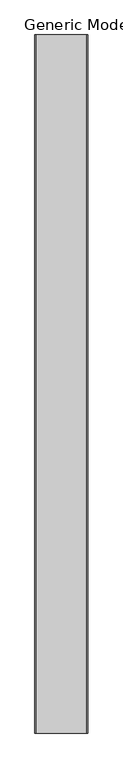
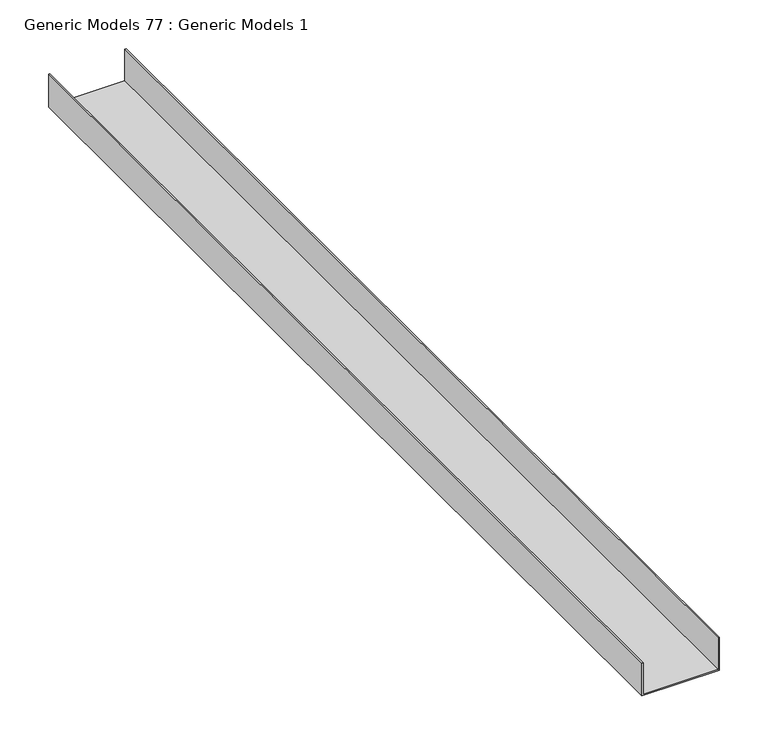
"""IFC4 building model written with IfcOpenShell, lengths in millimetres: proxy geometry, Generic Models 77 : Generic Models 1."""

from ifc_helpers import new_model, si_unit, frame, origin, place, context, project, spatial, polyline, outline, extrude, source, transform, mapped, element, save


def generic_models_77_generic_models_1_8efd1fd8(model_context):
    return source(origin(), model_context, "Body", "SweptSolid", [
        extrude(outline(polyline([(-225.976067, 46935.8735531), (-184.701067, 46935.8735531), (-184.701067, 46934.2860531), (-224.388567, 46934.2860531), (-224.388567, 46845.3860531), (-184.701067, 46845.3860531), (-184.701067, 46843.7985531), (-225.976067, 46843.7985531), (-225.976067, 46935.8735531)])), frame((0.0, 0.0, 0.0), z_axis=(0.0, 1.0, 0.0), x_axis=(0.0, 0.0, 1.0)), (0.0, 0.0, 1.0), 1219.2),
    ])


if __name__ == "__main__":
    model = new_model("IFC4")
    model_context = context("Model", 3, world=origin())
    ifc_project = project(units=[si_unit("LENGTHUNIT", "METRE", prefix="MILLI")], contexts=[model_context])
    site = spatial("IfcSite", under=ifc_project)
    building = spatial("IfcBuilding", under=site)
    placement = place(None, origin())
    generic_models_77_generic_models_1_shape = generic_models_77_generic_models_1_8efd1fd8(model_context)
    element("IfcBuildingElementProxy", 1, Name="Generic Models 77 : Generic Models 1", ObjectType="Generic Models 77 : Generic Models 1", at=placement, inside=building, context=model_context, shape_type="MappedRepresentation", body=[
        mapped(generic_models_77_generic_models_1_shape, transform((0.0, 0.0, 0.0), x_axis=(1.0, 0.0, 0.0), y_axis=(0.0, 1.0, 0.0), z_axis=(0.0, 0.0, 1.0))),
    ])
    save(model, "model.ifc")

# Revit data of these elements
# Element 1 (IfcBuildingElementProxy, "Generic Models 77 : Generic Models 1")
#   Materials on its faces: "METAL RUNNER CHANNEL; FASTEN @ 24\" O.C."
# Materials
#   "METAL RUNNER CHANNEL; FASTEN @ 24\" O.C.": class "Unassigned", colour RGB 210 209 208, transparency 0, Keynote = "M05121300.02", Cost = 0
